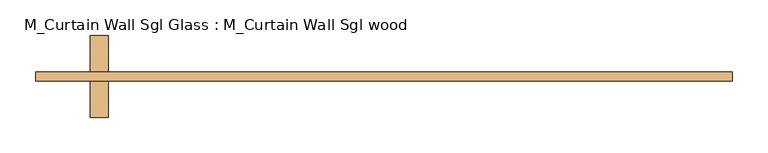
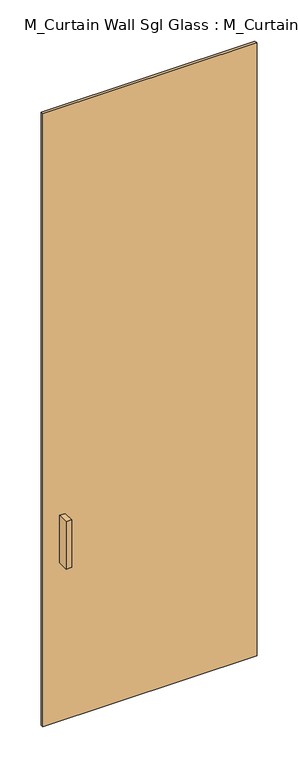
"""IFC4 building model written with IfcOpenShell, lengths in millimetres: door geometry, M_Curtain Wall Sgl Glass : M_Curtain Wall Sgl wood."""

from ifc_helpers import new_model, si_unit, frame, origin, origin_with_axes, place, context, project, spatial, polyline, outline, extrude, source, transform, mapped, element, save


def m_curtain_wall_sgl_glass_m_curtain_wall_sgl_wood_adc94a5f(model_context):
    return source(origin(), model_context, "Body", "SweptSolid", [
        extrude(outline(polyline([(-385.9, -12.5), (-411.3, -12.5), (-411.3, 38.3), (-385.9, 38.3), (-385.9, -12.5)])), frame((0.0, 0.0, 762.0), z_axis=(0.0, 0.0, 1.0), x_axis=(1.0, 0.0, 0.0)), (0.0, 0.0, 1.0), 228.6),
        extrude(outline(polyline([(-411.3, 101.8), (-385.9, 101.8), (-385.9, 51.0), (-411.3, 51.0), (-411.3, 101.8)])), frame((0.0, 0.0, 762.0), z_axis=(0.0, 0.0, 1.0), x_axis=(1.0, 0.0, 0.0)), (0.0, 0.0, 1.0), 228.6),
        extrude(outline(polyline([(487.5, 51.0), (487.5, 38.3), (-487.5, 38.3), (-487.5, 51.0), (487.5, 51.0)])), origin_with_axes(), (0.0, 0.0, 1.0), 2950.0),
    ])


if __name__ == "__main__":
    model = new_model("IFC4")
    model_context = context("Model", 3, world=origin())
    ifc_project = project(units=[si_unit("LENGTHUNIT", "METRE", prefix="MILLI")], contexts=[model_context])
    site = spatial("IfcSite", under=ifc_project)
    building = spatial("IfcBuilding", under=site)
    placement = place(None, origin())
    m_curtain_wall_sgl_glass_m_curtain_wall_sgl_wood_shape = m_curtain_wall_sgl_glass_m_curtain_wall_sgl_wood_adc94a5f(model_context)
    element("IfcDoor", 1, ObjectType="M_Curtain Wall Sgl Glass : M_Curtain Wall Sgl wood", at=placement, inside=building, context=model_context, shape_type="MappedRepresentation", body=[
        mapped(m_curtain_wall_sgl_glass_m_curtain_wall_sgl_wood_shape, transform((0.0, 0.0, 0.0), x_axis=(1.0, 0.0, 0.0), y_axis=(0.0, 1.0, 0.0), z_axis=(0.0, 0.0, 1.0))),
    ])
    save(model, "model.ifc")

# Revit data of these elements
# Type "M_Curtain Wall Sgl Glass : M_Curtain Wall Sgl wood"
#   Model = "12345669"
#   Manufacturer = "Dublin Doors"
#   Description = "Single Wood Door"
#   Type Mark = "45"
#   Fire Rating = "60M"
#   COBie.Type.CreatedBy = "design@eagle.com"
#   COBie.Type.CreatedOn = "2016-09-13T05:47:35"
#   COBie.Type.Name = "Doors_M_Curtain Wall Sgl Glass_M_Curtain Wall Sgl wood"
#   COBie.Type.Category = "23-30 10 00 : Doors"
#   COBie.Type.Description = "Single Wood Door"
#   COBie.Type.Manufacturer = "Dublin Doors"
#   COBie.Type.ModelNumber = "12345669"
#   Construction Type Id = "opn-d36"
#   Analytic Construction = "Wood panel"
#   COBie.Type.ReplacementCost = 0
#   Offset = 51 mm
#   Heat Transfer Coefficient (U) = 3.8042 W/(m²·K)
#   COBie.Type = yes
#   Function = 1
#   Glazing Material = Door - Panel
#   Visual Light Transmittance = 0
#   Solar Heat Gain Coefficient = 0
# Element 1 (IfcDoor, "M_Curtain Wall Sgl Glass : M_Curtain Wall Sgl wood")
#   Materials on its faces: "Aluminum", "Door - Panel"
# Materials
#   "Door - Panel": class "Wood", colour RGB 210 159 95, transparency 0
#   "Aluminum": class "Metal", colour RGB 247 247 247, transparency 0, Description = "Aluminum 6061", Cost = 0
